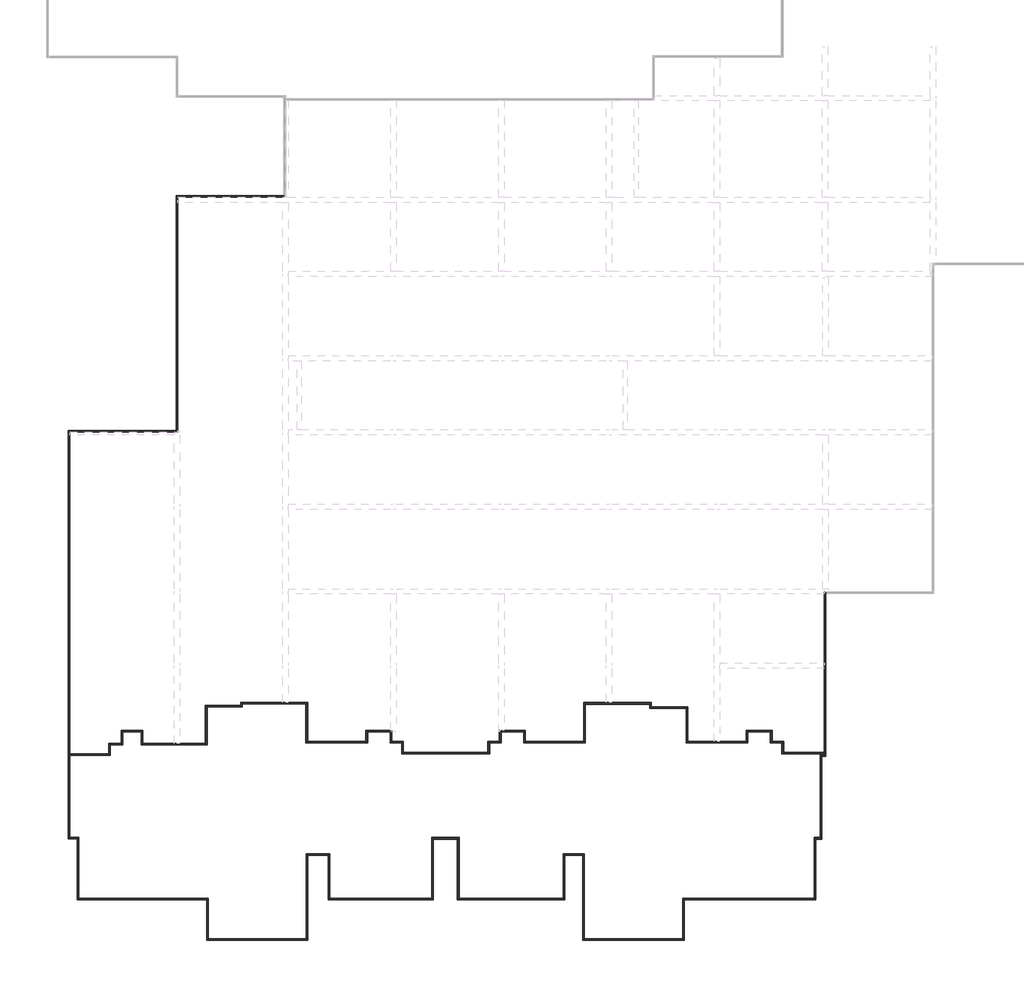
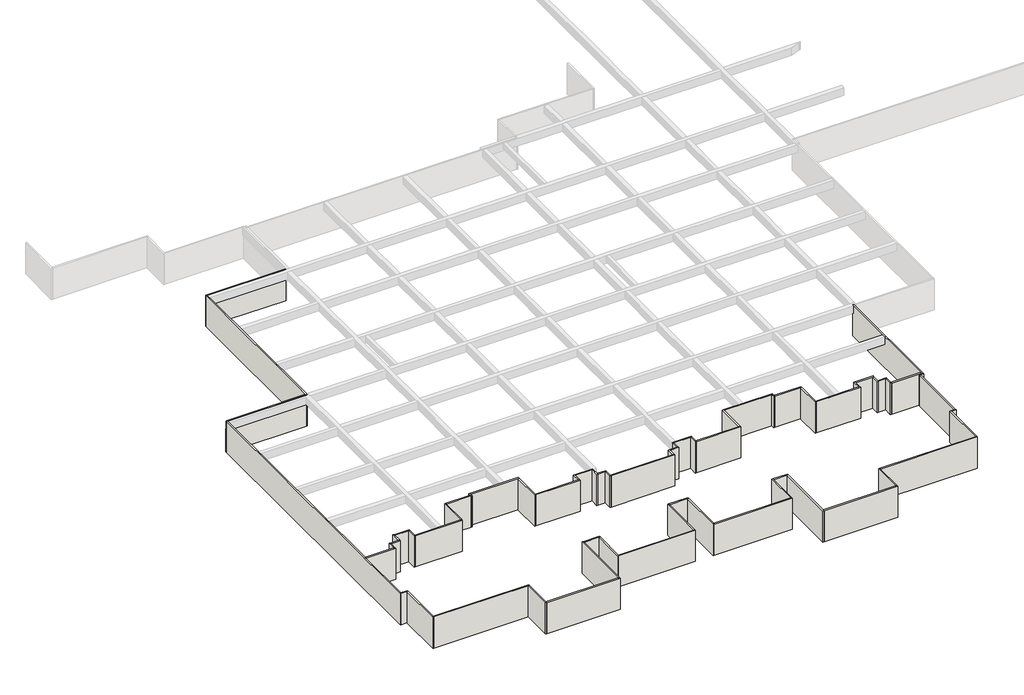
# One storey, part 1 of 14: 65 walls.
"""IFC4 building model written with IfcOpenShell, lengths in millimetres."""

from ifc_helpers import new_model, si_unit, origin, origin_with_axes, place, context, project, spatial, polyline, outline, extrude, faceted_brep, element, save

model = new_model("IFC4")

# Units and contexts
model_context = context("Model", 3, world=origin())
ifc_project = project(units=[si_unit("LENGTHUNIT", "METRE", prefix="MILLI")], contexts=[model_context])

# Site, building, storey
site = spatial("IfcSite", under=ifc_project)
building = spatial("IfcBuilding", under=site)
storey = spatial("IfcBuildingStorey", under=building, Name="户型图", Elevation=0.0)

# Walls
placement = place(None, origin())
element("IfcWall", 1, ObjectType="所有墙体", at=placement, inside=storey, context=model_context, shape_type="Brep", body=[
    faceted_brep([(-578191.2602569, -192711.2417661, 0.0), (-586191.2602569, -192711.2417661, 0.0), (-586191.2602569, -192711.2417661, 3300.0), (-578267.6529954, -192711.2417661, 3300.0), (-578191.2602569, -192711.2417661, 3300.0), (-578191.2602569, -192711.2417661, 2500.0), (-578191.2602569, -192831.2417661, 0.0), (-578191.2602569, -192831.2417661, 3300.0), (-578267.6529954, -192831.2417661, 3300.0), (-586071.2602569, -192831.2417661, 3300.0), (-586191.2602569, -192831.2417661, 3300.0), (-586191.2602569, -192831.2417661, 0.0), (-586071.2602569, -192831.2417661, 0.0)], [[[0, 1, 2, 3, 4, 5]], [[6, 7, 8, 9, 10, 11, 12]], [[1, 0, 6, 12, 11]], [[4, 3, 2, 10, 9, 8, 7]], [[0, 5, 4, 7, 6]], [[2, 1, 11, 10]]]),
])
element("IfcWall", 2, ObjectType="所有墙体", at=placement, inside=storey, context=model_context, shape_type="Brep", body=[
    faceted_brep([(-586191.2602569, -192831.2417661, 0.0), (-586191.2602569, -210132.8565135, 0.0), (-586191.2602569, -210252.8565135, 0.0), (-586191.2602569, -210252.8565135, 3300.0), (-586191.2602569, -210132.8565135, 3300.0), (-586191.2602569, -210092.8565135, 3300.0), (-586191.2602569, -192831.2417661, 3300.0), (-586071.2602569, -192831.2417661, 0.0), (-586071.2602569, -192831.2417661, 3300.0), (-586071.2602569, -210092.8565135, 3300.0), (-586071.2602569, -210132.8565135, 3300.0), (-586071.2602569, -210252.8565135, 3300.0), (-586071.2602569, -210252.8565135, 2500.0), (-586071.2602569, -210252.8565135, 0.0)], [[[0, 1, 2, 3, 4, 5, 6]], [[7, 8, 9, 10, 11, 12, 13]], [[2, 1, 0, 7, 13]], [[6, 5, 4, 3, 11, 10, 9, 8]], [[0, 6, 8, 7]], [[3, 2, 13, 12, 11]]]),
])
element("IfcWall", 3, ObjectType="所有墙体", at=placement, inside=storey, context=model_context, shape_type="Brep", body=[
    faceted_brep([(-586191.2602569, -210132.8565135, 0.0), (-594191.2602569, -210132.8565135, 0.0), (-594191.2602569, -210132.8565135, 3300.0), (-586191.2602569, -210132.8565135, 3300.0), (-586191.2602569, -210252.8565135, 0.0), (-586191.2602569, -210252.8565135, 3300.0), (-594071.2602569, -210252.8565135, 3300.0), (-594191.2602569, -210252.8565135, 3300.0), (-594191.2602569, -210252.8565135, 0.0), (-594071.2602569, -210252.8565135, 0.0)], [[[0, 1, 2, 3]], [[4, 5, 6, 7, 8, 9]], [[1, 0, 4, 9, 8]], [[3, 2, 7, 6, 5]], [[0, 3, 5, 4]], [[2, 1, 8, 7]]]),
])
element("IfcWall", 4, ObjectType="所有墙体", at=placement, inside=storey, context=model_context, shape_type="Brep", body=[
    faceted_brep([(-594191.2602569, -210252.8565135, 0.0), (-594191.2602569, -240452.8565135, 0.0), (-594191.2602569, -240452.8565135, 3300.0), (-594191.2602569, -210252.8565135, 3300.0), (-594071.2602569, -210252.8565135, 0.0), (-594071.2602569, -210252.8565135, 3300.0), (-594071.2602569, -234140.252781, 3300.0), (-594071.2602569, -234260.252781, 3300.0), (-594071.2602569, -240332.8565135, 3300.0), (-594071.2602569, -240452.8565135, 3300.0), (-594071.2602569, -240452.8565135, 0.0), (-594071.2602569, -240332.8565135, 0.0), (-594071.2602569, -234260.252781, 0.0), (-594071.2602569, -234140.252781, 0.0)], [[[0, 1, 2, 3]], [[4, 5, 6, 7, 8, 9, 10, 11, 12, 13]], [[1, 0, 4, 13, 12, 11, 10]], [[3, 2, 9, 8, 7, 6, 5]], [[0, 3, 5, 4]], [[2, 1, 10, 9]]]),
])
element("IfcWall", 5, ObjectType="所有墙体", at=placement, inside=storey, context=model_context, shape_type="Brep", body=[
    faceted_brep([(-594071.2602569, -240452.8565135, 0.0), (-593517.7604721, -240452.8565135, 0.0), (-593397.7604721, -240452.8565135, 0.0), (-593397.7604721, -240452.8565135, 3300.0), (-593517.7604721, -240452.8565135, 3300.0), (-594071.2602569, -240452.8565135, 3300.0), (-594071.2602569, -240332.8565135, 0.0), (-594071.2602569, -240332.8565135, 3300.0), (-593397.7604721, -240332.8565135, 3300.0), (-593397.7604721, -240332.8565135, 0.0)], [[[0, 1, 2, 3, 4, 5]], [[6, 7, 8, 9]], [[2, 1, 0, 6, 9]], [[5, 4, 3, 8, 7]], [[0, 5, 7, 6]], [[3, 2, 9, 8]]]),
])
element("IfcWall", 6, ObjectType="所有墙体", at=placement, inside=storey, context=model_context, shape_type="Brep", body=[
    faceted_brep([(-593517.7604721, -240452.8565135, 0.0), (-593517.7604721, -244961.010998, 0.0), (-593517.7604721, -244961.010998, 3300.0), (-593517.7604721, -240452.8565135, 3300.0), (-593397.7604721, -240452.8565135, 0.0), (-593397.7604721, -240452.8565135, 3300.0), (-593397.7604721, -244841.010998, 3300.0), (-593397.7604721, -244961.010998, 3300.0), (-593397.7604721, -244961.010998, 0.0), (-593397.7604721, -244841.010998, 0.0)], [[[0, 1, 2, 3]], [[4, 5, 6, 7, 8, 9]], [[1, 0, 4, 9, 8]], [[3, 2, 7, 6, 5]], [[0, 3, 5, 4]], [[2, 1, 8, 7]]]),
])
element("IfcWall", 7, ObjectType="所有墙体", at=placement, inside=storey, context=model_context, shape_type="Brep", body=[
    faceted_brep([(-593397.7604721, -244961.010998, 0.0), (-583922.7851213, -244961.010998, 0.0), (-583802.7851213, -244961.010998, 0.0), (-583802.7851213, -244961.010998, 3300.0), (-583922.7851213, -244961.010998, 3300.0), (-593397.7604721, -244961.010998, 3300.0), (-593397.7604721, -244841.010998, 0.0), (-593397.7604721, -244841.010998, 3300.0), (-583802.7851213, -244841.010998, 3300.0), (-583802.7851213, -244841.010998, 0.0)], [[[0, 1, 2, 3, 4, 5]], [[6, 7, 8, 9]], [[2, 1, 0, 6, 9]], [[5, 4, 3, 8, 7]], [[0, 5, 7, 6]], [[3, 2, 9, 8]]]),
])
element("IfcWall", 8, ObjectType="所有墙体", at=placement, inside=storey, context=model_context, shape_type="Brep", body=[
    faceted_brep([(-583922.7851213, -244961.010998, 0.0), (-583922.7851213, -247971.7198422, 0.0), (-583922.7851213, -247971.7198422, 3300.0), (-583922.7851213, -244961.010998, 3300.0), (-583802.7851213, -244961.010998, 0.0), (-583802.7851213, -244961.010998, 3300.0), (-583802.7851213, -247851.7198422, 3300.0), (-583802.7851213, -247971.7198422, 3300.0), (-583802.7851213, -247971.7198422, 0.0), (-583802.7851213, -247851.7198422, 0.0)], [[[0, 1, 2, 3]], [[4, 5, 6, 7, 8, 9]], [[1, 0, 4, 9, 8]], [[3, 2, 7, 6, 5]], [[0, 3, 5, 4]], [[2, 1, 8, 7]]]),
])
element("IfcWall", 9, ObjectType="所有墙体", at=placement, inside=storey, context=model_context, shape_type="Brep", body=[
    faceted_brep([(-583802.7851213, -247971.7198422, 0.0), (-576406.141893, -247971.7198422, 0.0), (-576406.141893, -247971.7198422, 3300.0), (-583802.7851213, -247971.7198422, 3300.0), (-583802.7851213, -247851.7198422, 0.0), (-583802.7851213, -247851.7198422, 3300.0), (-576526.141893, -247851.7198422, 3300.0), (-576406.141893, -247851.7198422, 3300.0), (-576406.141893, -247851.7198422, 0.0), (-576526.141893, -247851.7198422, 0.0)], [[[0, 1, 2, 3]], [[4, 5, 6, 7, 8, 9]], [[1, 0, 4, 9, 8]], [[3, 2, 7, 6, 5]], [[0, 3, 5, 4]], [[2, 1, 8, 7]]]),
])
element("IfcWall", 10, ObjectType="所有墙体", at=placement, inside=storey, context=model_context, shape_type="Brep", body=[
    faceted_brep([(-576406.141893, -247851.7198422, 0.0), (-576406.141893, -241679.9697972, 0.0), (-576406.141893, -241559.9697972, 0.0), (-576406.141893, -241559.9697972, 3300.0), (-576406.141893, -241679.9697972, 3300.0), (-576406.141893, -247851.7198422, 3300.0), (-576526.141893, -247851.7198422, 0.0), (-576526.141893, -247851.7198422, 3300.0), (-576526.141893, -241559.9697972, 3300.0), (-576526.141893, -241559.9697972, 0.0)], [[[0, 1, 2, 3, 4, 5]], [[6, 7, 8, 9]], [[2, 1, 0, 6, 9]], [[5, 4, 3, 8, 7]], [[0, 5, 7, 6]], [[3, 2, 9, 8]]]),
])
element("IfcWall", 11, ObjectType="所有墙体", at=placement, inside=storey, context=model_context, shape_type="Brep", body=[
    faceted_brep([(-576406.141893, -241679.9697972, 0.0), (-574919.1182202, -241679.9697972, 0.0), (-574799.1182202, -241679.9697972, 0.0), (-574799.1182202, -241679.9697972, 3300.0), (-574919.1182202, -241679.9697972, 3300.0), (-576406.141893, -241679.9697972, 3300.0), (-576406.141893, -241559.9697972, 0.0), (-576406.141893, -241559.9697972, 3300.0), (-574799.1182202, -241559.9697972, 3300.0), (-574799.1182202, -241559.9697972, 0.0)], [[[0, 1, 2, 3, 4, 5]], [[6, 7, 8, 9]], [[2, 1, 0, 6, 9]], [[5, 4, 3, 8, 7]], [[0, 5, 7, 6]], [[3, 2, 9, 8]]]),
])
element("IfcWall", 12, ObjectType="所有墙体", at=placement, inside=storey, context=model_context, shape_type="Brep", body=[
    faceted_brep([(-574919.1182202, -241679.9697972, 0.0), (-574919.1182202, -244961.010998, 0.0), (-574919.1182202, -244961.010998, 3300.0), (-574919.1182202, -241679.9697972, 3300.0), (-574799.1182202, -241679.9697972, 0.0), (-574799.1182202, -241679.9697972, 3300.0), (-574799.1182202, -244841.010998, 3300.0), (-574799.1182202, -244961.010998, 3300.0), (-574799.1182202, -244961.010998, 0.0), (-574799.1182202, -244841.010998, 0.0)], [[[0, 1, 2, 3]], [[4, 5, 6, 7, 8, 9]], [[1, 0, 4, 9, 8]], [[3, 2, 7, 6, 5]], [[0, 3, 5, 4]], [[2, 1, 8, 7]]]),
])
element("IfcWall", 13, ObjectType="所有墙体", at=placement, inside=storey, context=model_context, shape_type="Brep", body=[
    faceted_brep([(-574799.1182202, -244961.010998, 0.0), (-567099.1182202, -244961.010998, 0.0), (-567099.1182202, -244961.010998, 3300.0), (-574799.1182202, -244961.010998, 3300.0), (-574799.1182202, -244841.010998, 0.0), (-574799.1182202, -244841.010998, 3300.0), (-567219.1182202, -244841.010998, 3300.0), (-567099.1182202, -244841.010998, 3300.0), (-567099.1182202, -244841.010998, 0.0), (-567219.1182202, -244841.010998, 0.0)], [[[0, 1, 2, 3]], [[4, 5, 6, 7, 8, 9]], [[1, 0, 4, 9, 8]], [[3, 2, 7, 6, 5]], [[0, 3, 5, 4]], [[2, 1, 8, 7]]]),
])
element("IfcWall", 14, ObjectType="所有墙体", at=placement, inside=storey, context=model_context, shape_type="Brep", body=[
    faceted_brep([(-567099.1182202, -244841.010998, 0.0), (-567099.1182202, -240461.010998, 0.0), (-567099.1182202, -240341.010998, 0.0), (-567099.1182202, -240341.010998, 3300.0), (-567099.1182202, -240461.010998, 3300.0), (-567099.1182202, -244841.010998, 3300.0), (-567219.1182202, -244841.010998, 0.0), (-567219.1182202, -244841.010998, 3300.0), (-567219.1182202, -240341.010998, 3300.0), (-567219.1182202, -240341.010998, 0.0)], [[[0, 1, 2, 3, 4, 5]], [[6, 7, 8, 9]], [[2, 1, 0, 6, 9]], [[5, 4, 3, 8, 7]], [[0, 5, 7, 6]], [[3, 2, 9, 8]]]),
])
element("IfcWall", 15, ObjectType="所有墙体", at=placement, inside=storey, context=model_context, shape_type="Brep", body=[
    faceted_brep([(-567099.1182202, -240461.010998, 0.0), (-565319.1182202, -240461.010998, 0.0), (-565199.1182202, -240461.010998, 0.0), (-565199.1182202, -240461.010998, 3300.0), (-565319.1182202, -240461.010998, 3300.0), (-567099.1182202, -240461.010998, 3300.0), (-567099.1182202, -240341.010998, 0.0), (-567099.1182202, -240341.010998, 3300.0), (-565199.1182202, -240341.010998, 3300.0), (-565199.1182202, -240341.010998, 0.0)], [[[0, 1, 2, 3, 4, 5]], [[6, 7, 8, 9]], [[2, 1, 0, 6, 9]], [[5, 4, 3, 8, 7]], [[0, 5, 7, 6]], [[3, 2, 9, 8]]]),
])
element("IfcWall", 16, ObjectType="所有墙体", at=placement, inside=storey, context=model_context, shape_type="Brep", body=[
    faceted_brep([(-565319.1182202, -240461.010998, 0.0), (-565319.1182202, -244961.010998, 0.0), (-565319.1182202, -244961.010998, 3300.0), (-565319.1182202, -240461.010998, 3300.0), (-565199.1182202, -240461.010998, 0.0), (-565199.1182202, -240461.010998, 3300.0), (-565199.1182202, -244841.010998, 3300.0), (-565199.1182202, -244961.010998, 3300.0), (-565199.1182202, -244961.010998, 0.0), (-565199.1182202, -244841.010998, 0.0)], [[[0, 1, 2, 3]], [[4, 5, 6, 7, 8, 9]], [[1, 0, 4, 9, 8]], [[3, 2, 7, 6, 5]], [[0, 3, 5, 4]], [[2, 1, 8, 7]]]),
])
element("IfcWall", 17, ObjectType="所有墙体", at=placement, inside=storey, context=model_context, shape_type="Brep", body=[
    faceted_brep([(-565199.1182202, -244961.010998, 0.0), (-557352.768648, -244961.010998, 0.0), (-557352.768648, -244961.010998, 3300.0), (-565199.1182202, -244961.010998, 3300.0), (-565199.1182202, -244841.010998, 0.0), (-565199.1182202, -244841.010998, 3300.0), (-557472.768648, -244841.010998, 3300.0), (-557352.768648, -244841.010998, 3300.0), (-557352.768648, -244841.010998, 0.0), (-557472.768648, -244841.010998, 0.0)], [[[0, 1, 2, 3]], [[4, 5, 6, 7, 8, 9]], [[1, 0, 4, 9, 8]], [[3, 2, 7, 6, 5]], [[0, 3, 5, 4]], [[2, 1, 8, 7]]]),
])
element("IfcWall", 18, ObjectType="所有墙体", at=placement, inside=storey, context=model_context, shape_type="Brep", body=[
    faceted_brep([(-557352.768648, -244841.010998, 0.0), (-557352.768648, -241679.9697972, 0.0), (-557352.768648, -241559.9697972, 0.0), (-557352.768648, -241559.9697972, 3300.0), (-557352.768648, -241679.9697972, 3300.0), (-557352.768648, -244841.010998, 3300.0), (-557472.768648, -244841.010998, 0.0), (-557472.768648, -244841.010998, 3300.0), (-557472.768648, -241559.9697972, 3300.0), (-557472.768648, -241559.9697972, 0.0)], [[[0, 1, 2, 3, 4, 5]], [[6, 7, 8, 9]], [[2, 1, 0, 6, 9]], [[5, 4, 3, 8, 7]], [[0, 5, 7, 6]], [[3, 2, 9, 8]]]),
])
element("IfcWall", 19, ObjectType="所有墙体", at=placement, inside=storey, context=model_context, shape_type="Brep", body=[
    faceted_brep([(-557352.768648, -241679.9697972, 0.0), (-556019.1064476, -241679.9697972, 0.0), (-555899.1064476, -241679.9697972, 0.0), (-555899.1064476, -241679.9697972, 3300.0), (-556019.1064476, -241679.9697972, 3300.0), (-557352.768648, -241679.9697972, 3300.0), (-557352.768648, -241559.9697972, 0.0), (-557352.768648, -241559.9697972, 3300.0), (-555899.1064476, -241559.9697972, 3300.0), (-555899.1064476, -241559.9697972, 0.0)], [[[0, 1, 2, 3, 4, 5]], [[6, 7, 8, 9]], [[2, 1, 0, 6, 9]], [[5, 4, 3, 8, 7]], [[0, 5, 7, 6]], [[3, 2, 9, 8]]]),
])
element("IfcWall", 20, ObjectType="所有墙体", at=placement, inside=storey, context=model_context, shape_type="Brep", body=[
    faceted_brep([(-556019.1064476, -241679.9697972, 0.0), (-556019.1064476, -247971.7198422, 0.0), (-556019.1064476, -247971.7198422, 3300.0), (-556019.1064476, -241679.9697972, 3300.0), (-555899.1064476, -241679.9697972, 0.0), (-555899.1064476, -241679.9697972, 3300.0), (-555899.1064476, -247851.7198422, 3300.0), (-555899.1064476, -247971.7198422, 3300.0), (-555899.1064476, -247971.7198422, 0.0), (-555899.1064476, -247851.7198422, 0.0)], [[[0, 1, 2, 3]], [[4, 5, 6, 7, 8, 9]], [[1, 0, 4, 9, 8]], [[3, 2, 7, 6, 5]], [[0, 3, 5, 4]], [[2, 1, 8, 7]]]),
])
element("IfcWall", 21, ObjectType="所有墙体", at=placement, inside=storey, context=model_context, shape_type="Brep", body=[
    faceted_brep([(-555899.1064476, -247971.7198422, 0.0), (-548506.1227729, -247971.7198422, 0.0), (-548506.1227729, -247971.7198422, 3300.0), (-555899.1064476, -247971.7198422, 3300.0), (-555899.1064476, -247851.7198422, 0.0), (-555899.1064476, -247851.7198422, 3300.0), (-548626.1227729, -247851.7198422, 3300.0), (-548506.1227729, -247851.7198422, 3300.0), (-548506.1227729, -247851.7198422, 0.0), (-548626.1227729, -247851.7198422, 0.0)], [[[0, 1, 2, 3]], [[4, 5, 6, 7, 8, 9]], [[1, 0, 4, 9, 8]], [[3, 2, 7, 6, 5]], [[0, 3, 5, 4]], [[2, 1, 8, 7]]]),
])
element("IfcWall", 22, ObjectType="所有墙体", at=placement, inside=storey, context=model_context, shape_type="Brep", body=[
    faceted_brep([(-548506.1227729, -247851.7198422, 0.0), (-548506.1227729, -244961.010998, 0.0), (-548506.1227729, -244841.010998, 0.0), (-548506.1227729, -244841.010998, 3300.0), (-548506.1227729, -244961.010998, 3300.0), (-548506.1227729, -247851.7198422, 3300.0), (-548626.1227729, -247851.7198422, 0.0), (-548626.1227729, -247851.7198422, 3300.0), (-548626.1227729, -244841.010998, 3300.0), (-548626.1227729, -244841.010998, 0.0)], [[[0, 1, 2, 3, 4, 5]], [[6, 7, 8, 9]], [[2, 1, 0, 6, 9]], [[5, 4, 3, 8, 7]], [[0, 5, 7, 6]], [[3, 2, 9, 8]]]),
])
element("IfcWall", 23, ObjectType="所有墙体", at=placement, inside=storey, context=model_context, shape_type="Brep", body=[
    faceted_brep([(-548506.1227729, -244961.010998, 0.0), (-538752.7570659, -244961.010998, 0.0), (-538752.7570659, -244961.010998, 3300.0), (-548506.1227729, -244961.010998, 3300.0), (-548506.1227729, -244841.010998, 0.0), (-548506.1227729, -244841.010998, 3300.0), (-538872.7570659, -244841.010998, 3300.0), (-538752.7570659, -244841.010998, 3300.0), (-538752.7570659, -244841.010998, 0.0), (-538872.7570659, -244841.010998, 0.0)], [[[0, 1, 2, 3]], [[4, 5, 6, 7, 8, 9]], [[1, 0, 4, 9, 8]], [[3, 2, 7, 6, 5]], [[0, 3, 5, 4]], [[2, 1, 8, 7]]]),
])
element("IfcWall", 24, ObjectType="所有墙体", at=placement, inside=storey, context=model_context, shape_type="Brep", body=[
    faceted_brep([(-538752.7570659, -244841.010998, 0.0), (-538752.7570659, -240461.010998, 0.0), (-538752.7570659, -240341.010998, 0.0), (-538752.7570659, -240341.010998, 3300.0), (-538752.7570659, -240461.010998, 3300.0), (-538752.7570659, -244841.010998, 3300.0), (-538872.7570659, -244841.010998, 0.0), (-538872.7570659, -244841.010998, 3300.0), (-538872.7570659, -240341.010998, 3300.0), (-538872.7570659, -240341.010998, 0.0)], [[[0, 1, 2, 3, 4, 5]], [[6, 7, 8, 9]], [[2, 1, 0, 6, 9]], [[5, 4, 3, 8, 7]], [[0, 5, 7, 6]], [[3, 2, 9, 8]]]),
])
element("IfcWall", 25, ObjectType="所有墙体", at=placement, inside=storey, context=model_context, shape_type="Brep", body=[
    faceted_brep([(-538752.7570659, -240461.010998, 0.0), (-538297.7352575, -240461.010998, 0.0), (-538297.7352575, -240461.010998, 3300.0), (-538752.7570659, -240461.010998, 3300.0), (-538752.7570659, -240341.010998, 0.0), (-538752.7570659, -240341.010998, 3300.0), (-538417.7352575, -240341.010998, 3300.0), (-538297.7352575, -240341.010998, 3300.0), (-538297.7352575, -240341.010998, 0.0), (-538417.7352575, -240341.010998, 0.0)], [[[0, 1, 2, 3]], [[4, 5, 6, 7, 8, 9]], [[1, 0, 4, 9, 8]], [[3, 2, 7, 6, 5]], [[0, 3, 5, 4]], [[2, 1, 8, 7]]]),
])
element("IfcWall", 26, ObjectType="所有墙体", at=placement, inside=storey, context=model_context, shape_type="SweptSolid", body=[
    extrude(outline(polyline([(-538297.7352575, -234322.4901809), (-538297.7352575, -240341.010998), (-538417.7352575, -240341.010998), (-538417.7352575, -234322.4901809), (-538297.7352575, -234322.4901809)])), origin_with_axes(), (0.0, 0.0, 1.0), 3300.0),
])
element("IfcWall", 27, ObjectType="所有墙体", at=placement, inside=storey, context=model_context, shape_type="Brep", body=[
    faceted_brep([(-538417.7352575, -234322.4901809, 0.0), (-538297.7352575, -234322.4901809, 0.0), (-537997.7352575, -234322.4901809, 0.0), (-537997.7352575, -234322.4901809, 3300.0), (-538297.7352575, -234322.4901809, 3300.0), (-538417.7352575, -234322.4901809, 3300.0), (-538417.7352575, -234202.4901809, 0.0), (-538417.7352575, -234202.4901809, 3300.0), (-538117.7352575, -234202.4901809, 3300.0), (-537997.7352575, -234202.4901809, 3300.0), (-537997.7352575, -234202.4901809, 0.0), (-538117.7352575, -234202.4901809, 0.0)], [[[0, 1, 2, 3, 4, 5]], [[6, 7, 8, 9, 10, 11]], [[2, 1, 0, 6, 11, 10]], [[5, 4, 3, 9, 8, 7]], [[0, 5, 7, 6]], [[3, 2, 10, 9]]]),
])
element("IfcWall", 28, ObjectType="所有墙体", at=placement, inside=storey, context=model_context, shape_type="Brep", body=[
    faceted_brep([(-537997.7352575, -234202.4901809, 0.0), (-537997.7352575, -222250.9174567, 0.0), (-537997.7352575, -222130.9174567, 0.0), (-537997.7352575, -222130.9174567, 3300.0), (-537997.7352575, -222250.9174567, 3300.0), (-537997.7352575, -222292.8565135, 3300.0), (-537997.7352575, -234202.4901809, 3300.0), (-538117.7352575, -234202.4901809, 0.0), (-538117.7352575, -234202.4901809, 3300.0), (-538117.7352575, -234137.8504047, 3300.0), (-538117.7352575, -234017.8504047, 3300.0), (-538117.7352575, -222292.8565135, 3300.0), (-538117.7352575, -222130.9174567, 3300.0), (-538117.7352575, -222130.9174567, 2500.0), (-538117.7352575, -222130.9174567, 0.0), (-538117.7352575, -234017.8504047, 0.0), (-538117.7352575, -234137.8504047, 0.0)], [[[0, 1, 2, 3, 4, 5, 6]], [[7, 8, 9, 10, 11, 12, 13, 14, 15, 16]], [[2, 1, 0, 7, 16, 15, 14]], [[6, 5, 4, 3, 12, 11, 10, 9, 8]], [[0, 6, 8, 7]], [[3, 2, 14, 13, 12]]]),
])
element("IfcWall", 29, ObjectType="所有墙体", at=placement, inside=storey, context=model_context, shape_type="Brep", body=[
    faceted_brep([(-594071.2602569, -234260.252781, 0.0), (-591071.2602569, -234260.252781, 0.0), (-591071.2602569, -234260.252781, 3300.0), (-594071.2602569, -234260.252781, 3300.0), (-594071.2602569, -234140.252781, 0.0), (-594071.2602569, -234140.252781, 3300.0), (-591191.2602569, -234140.252781, 3300.0), (-591071.2602569, -234140.252781, 3300.0), (-591071.2602569, -234140.252781, 0.0), (-591191.2602569, -234140.252781, 0.0)], [[[0, 1, 2, 3]], [[4, 5, 6, 7, 8, 9]], [[1, 0, 4, 9, 8]], [[3, 2, 7, 6, 5]], [[0, 3, 5, 4]], [[2, 1, 8, 7]]]),
])
element("IfcWall", 30, ObjectType="所有墙体", at=placement, inside=storey, context=model_context, shape_type="Brep", body=[
    faceted_brep([(-591071.2602569, -234140.252781, 0.0), (-591071.2602569, -233463.599968, 0.0), (-591071.2602569, -233343.599968, 0.0), (-591071.2602569, -233343.599968, 3300.0), (-591071.2602569, -233463.599968, 3300.0), (-591071.2602569, -234140.252781, 3300.0), (-591191.2602569, -234140.252781, 0.0), (-591191.2602569, -234140.252781, 3300.0), (-591191.2602569, -233343.599968, 3300.0), (-591191.2602569, -233343.599968, 0.0)], [[[0, 1, 2, 3, 4, 5]], [[6, 7, 8, 9]], [[2, 1, 0, 6, 9]], [[5, 4, 3, 8, 7]], [[0, 5, 7, 6]], [[3, 2, 9, 8]]]),
])
element("IfcWall", 31, ObjectType="所有墙体", at=placement, inside=storey, context=model_context, shape_type="Brep", body=[
    faceted_brep([(-591071.2602569, -233463.599968, 0.0), (-590139.9591732, -233463.599968, 0.0), (-590139.9591732, -233463.599968, 3300.0), (-591071.2602569, -233463.599968, 3300.0), (-591071.2602569, -233343.599968, 0.0), (-591071.2602569, -233343.599968, 3300.0), (-590259.9591732, -233343.599968, 3300.0), (-590139.9591732, -233343.599968, 3300.0), (-590139.9591732, -233343.599968, 0.0), (-590259.9591732, -233343.599968, 0.0)], [[[0, 1, 2, 3]], [[4, 5, 6, 7, 8, 9]], [[1, 0, 4, 9, 8]], [[3, 2, 7, 6, 5]], [[0, 3, 5, 4]], [[2, 1, 8, 7]]]),
])
element("IfcWall", 32, ObjectType="所有墙体", at=placement, inside=storey, context=model_context, shape_type="Brep", body=[
    faceted_brep([(-590139.9591732, -233343.599968, 0.0), (-590139.9591732, -232514.6386108, 0.0), (-590139.9591732, -232394.6386108, 0.0), (-590139.9591732, -232394.6386108, 3300.0), (-590139.9591732, -232514.6386108, 3300.0), (-590139.9591732, -233343.599968, 3300.0), (-590259.9591732, -233343.599968, 0.0), (-590259.9591732, -233343.599968, 3300.0), (-590259.9591732, -232394.6386108, 3300.0), (-590259.9591732, -232394.6386108, 0.0)], [[[0, 1, 2, 3, 4, 5]], [[6, 7, 8, 9]], [[2, 1, 0, 6, 9]], [[5, 4, 3, 8, 7]], [[0, 5, 7, 6]], [[3, 2, 9, 8]]]),
])
element("IfcWall", 33, ObjectType="所有墙体", at=placement, inside=storey, context=model_context, shape_type="Brep", body=[
    faceted_brep([(-590139.9591732, -232514.6386108, 0.0), (-588758.8992985, -232514.6386108, 0.0), (-588638.8992985, -232514.6386108, 0.0), (-588638.8992985, -232514.6386108, 3300.0), (-588758.8992985, -232514.6386108, 3300.0), (-590139.9591732, -232514.6386108, 3300.0), (-590139.9591732, -232394.6386108, 0.0), (-590139.9591732, -232394.6386108, 3300.0), (-588638.8992985, -232394.6386108, 3300.0), (-588638.8992985, -232394.6386108, 0.0)], [[[0, 1, 2, 3, 4, 5]], [[6, 7, 8, 9]], [[2, 1, 0, 6, 9]], [[5, 4, 3, 8, 7]], [[0, 5, 7, 6]], [[3, 2, 9, 8]]]),
])
element("IfcWall", 34, ObjectType="所有墙体", at=placement, inside=storey, context=model_context, shape_type="Brep", body=[
    faceted_brep([(-588758.8992985, -232514.6386108, 0.0), (-588758.8992985, -233463.599968, 0.0), (-588758.8992985, -233463.599968, 3300.0), (-588758.8992985, -232514.6386108, 3300.0), (-588638.8992985, -232514.6386108, 0.0), (-588638.8992985, -232514.6386108, 3300.0), (-588638.8992985, -233343.599968, 3300.0), (-588638.8992985, -233463.599968, 3300.0), (-588638.8992985, -233463.599968, 0.0), (-588638.8992985, -233343.599968, 0.0)], [[[0, 1, 2, 3]], [[4, 5, 6, 7, 8, 9]], [[1, 0, 4, 9, 8]], [[3, 2, 7, 6, 5]], [[0, 3, 5, 4]], [[2, 1, 8, 7]]]),
])
element("IfcWall", 35, ObjectType="所有墙体", at=placement, inside=storey, context=model_context, shape_type="Brep", body=[
    faceted_brep([(-588638.8992985, -233463.599968, 0.0), (-583889.9552825, -233463.599968, 0.0), (-583889.9552825, -233463.599968, 3300.0), (-588638.8992985, -233463.599968, 3300.0), (-588638.8992985, -233343.599968, 0.0), (-588638.8992985, -233343.599968, 3300.0), (-584009.9552825, -233343.599968, 3300.0), (-583889.9552825, -233343.599968, 3300.0), (-583889.9552825, -233343.599968, 0.0), (-584009.9552825, -233343.599968, 0.0)], [[[0, 1, 2, 3]], [[4, 5, 6, 7, 8, 9]], [[1, 0, 4, 9, 8]], [[3, 2, 7, 6, 5]], [[0, 3, 5, 4]], [[2, 1, 8, 7]]]),
])
element("IfcWall", 36, ObjectType="所有墙体", at=placement, inside=storey, context=model_context, shape_type="Brep", body=[
    faceted_brep([(-583889.9552825, -233343.599968, 0.0), (-583889.9552825, -230671.6117982, 0.0), (-583889.9552825, -230551.6117982, 0.0), (-583889.9552825, -230551.6117982, 3300.0), (-583889.9552825, -230671.6117982, 3300.0), (-583889.9552825, -233343.599968, 3300.0), (-584009.9552825, -233343.599968, 0.0), (-584009.9552825, -233343.599968, 3300.0), (-584009.9552825, -230551.6117982, 3300.0), (-584009.9552825, -230551.6117982, 0.0)], [[[0, 1, 2, 3, 4, 5]], [[6, 7, 8, 9]], [[2, 1, 0, 6, 9]], [[5, 4, 3, 8, 7]], [[0, 5, 7, 6]], [[3, 2, 9, 8]]]),
])
element("IfcWall", 37, ObjectType="所有墙体", at=placement, inside=storey, context=model_context, shape_type="SweptSolid", body=[
    extrude(outline(polyline([(-581406.838098, -230671.6117982), (-583889.9552825, -230671.6117982), (-583889.9552825, -230551.6117982), (-581406.838098, -230551.6117982), (-581406.838098, -230671.6117982)])), origin_with_axes(), (0.0, 0.0, 1.0), 3300.0),
])
element("IfcWall", 38, ObjectType="所有墙体", at=placement, inside=storey, context=model_context, shape_type="Brep", body=[
    faceted_brep([(-581286.838098, -230671.6117982, 0.0), (-581286.838098, -230424.5164481, 0.0), (-581286.838098, -230304.5164481, 0.0), (-581286.838098, -230304.5164481, 3300.0), (-581286.838098, -230424.5164481, 3300.0), (-581286.838098, -230671.6117982, 3300.0), (-581406.838098, -230671.6117982, 0.0), (-581406.838098, -230671.6117982, 3300.0), (-581406.838098, -230551.6117982, 3300.0), (-581406.838098, -230304.5164481, 3300.0), (-581406.838098, -230304.5164481, 0.0), (-581406.838098, -230551.6117982, 0.0)], [[[0, 1, 2, 3, 4, 5]], [[6, 7, 8, 9, 10, 11]], [[2, 1, 0, 6, 11, 10]], [[5, 4, 3, 9, 8, 7]], [[0, 5, 7, 6]], [[3, 2, 10, 9]]]),
])
element("IfcWall", 39, ObjectType="所有墙体", at=placement, inside=storey, context=model_context, shape_type="Brep", body=[
    faceted_brep([(-581286.838098, -230424.5164481, 0.0), (-576556.5593395, -230424.5164481, 0.0), (-576436.5593395, -230424.5164481, 0.0), (-576436.5593395, -230424.5164481, 3300.0), (-576556.5593395, -230424.5164481, 3300.0), (-581286.838098, -230424.5164481, 3300.0), (-581286.838098, -230304.5164481, 0.0), (-581286.838098, -230304.5164481, 3300.0), (-576436.5593395, -230304.5164481, 3300.0), (-576436.5593395, -230304.5164481, 0.0)], [[[0, 1, 2, 3, 4, 5]], [[6, 7, 8, 9]], [[2, 1, 0, 6, 9]], [[5, 4, 3, 8, 7]], [[0, 5, 7, 6]], [[3, 2, 9, 8]]]),
])
element("IfcWall", 40, ObjectType="所有墙体", at=placement, inside=storey, context=model_context, shape_type="Brep", body=[
    faceted_brep([(-576556.5593395, -230424.5164481, 0.0), (-576556.5593395, -233329.9306648, 0.0), (-576556.5593395, -233329.9306648, 3300.0), (-576556.5593395, -230424.5164481, 3300.0), (-576436.5593395, -230424.5164481, 0.0), (-576436.5593395, -230424.5164481, 3300.0), (-576436.5593395, -233209.9306648, 3300.0), (-576436.5593395, -233329.9306648, 3300.0), (-576436.5593395, -233329.9306648, 0.0), (-576436.5593395, -233209.9306648, 0.0)], [[[0, 1, 2, 3]], [[4, 5, 6, 7, 8, 9]], [[1, 0, 4, 9, 8]], [[3, 2, 7, 6, 5]], [[0, 3, 5, 4]], [[2, 1, 8, 7]]]),
])
element("IfcWall", 41, ObjectType="所有墙体", at=placement, inside=storey, context=model_context, shape_type="Brep", body=[
    faceted_brep([(-576436.5593395, -233329.9306648, 0.0), (-571989.7987118, -233329.9306648, 0.0), (-571989.7987118, -233329.9306648, 3300.0), (-576436.5593395, -233329.9306648, 3300.0), (-576436.5593395, -233209.9306648, 0.0), (-576436.5593395, -233209.9306648, 3300.0), (-572109.7987118, -233209.9306648, 3300.0), (-571989.7987118, -233209.9306648, 3300.0), (-571989.7987118, -233209.9306648, 0.0), (-572109.7987118, -233209.9306648, 0.0)], [[[0, 1, 2, 3]], [[4, 5, 6, 7, 8, 9]], [[1, 0, 4, 9, 8]], [[3, 2, 7, 6, 5]], [[0, 3, 5, 4]], [[2, 1, 8, 7]]]),
])
element("IfcWall", 42, ObjectType="所有墙体", at=placement, inside=storey, context=model_context, shape_type="Brep", body=[
    faceted_brep([(-571989.7987118, -233209.9306648, 0.0), (-571989.7987118, -232514.6386108, 0.0), (-571989.7987118, -232394.6386108, 0.0), (-571989.7987118, -232394.6386108, 3300.0), (-571989.7987118, -232514.6386108, 3300.0), (-571989.7987118, -233209.9306648, 3300.0), (-572109.7987118, -233209.9306648, 0.0), (-572109.7987118, -233209.9306648, 3300.0), (-572109.7987118, -232394.6386108, 3300.0), (-572109.7987118, -232394.6386108, 0.0)], [[[0, 1, 2, 3, 4, 5]], [[6, 7, 8, 9]], [[2, 1, 0, 6, 9]], [[5, 4, 3, 8, 7]], [[0, 5, 7, 6]], [[3, 2, 9, 8]]]),
])
element("IfcWall", 43, ObjectType="所有墙体", at=placement, inside=storey, context=model_context, shape_type="Brep", body=[
    faceted_brep([(-571989.7987118, -232514.6386108, 0.0), (-570308.8878112, -232514.6386108, 0.0), (-570188.8878112, -232514.6386108, 0.0), (-570188.8878112, -232514.6386108, 3300.0), (-570308.8878112, -232514.6386108, 3300.0), (-571989.7987118, -232514.6386108, 3300.0), (-571989.7987118, -232394.6386108, 0.0), (-571989.7987118, -232394.6386108, 3300.0), (-570267.6529954, -232394.6386108, 3300.0), (-570188.8878112, -232394.6386108, 3300.0), (-570188.8878112, -232394.6386108, 2500.0), (-570188.8878112, -232394.6386108, 0.0)], [[[0, 1, 2, 3, 4, 5]], [[6, 7, 8, 9, 10, 11]], [[2, 1, 0, 6, 11]], [[5, 4, 3, 9, 8, 7]], [[0, 5, 7, 6]], [[3, 2, 11, 10, 9]]]),
])
element("IfcWall", 44, ObjectType="所有墙体", at=placement, inside=storey, context=model_context, shape_type="Brep", body=[
    faceted_brep([(-570308.8878112, -232514.6386108, 0.0), (-570308.8878112, -233329.9306648, 0.0), (-570308.8878112, -233329.9306648, 3300.0), (-570308.8878112, -232514.6386108, 3300.0), (-570188.8878112, -232514.6386108, 0.0), (-570188.8878112, -232514.6386108, 3300.0), (-570188.8878112, -233209.9306648, 3300.0), (-570188.8878112, -233329.9306648, 3300.0), (-570188.8878112, -233329.9306648, 0.0), (-570188.8878112, -233209.9306648, 0.0)], [[[0, 1, 2, 3]], [[4, 5, 6, 7, 8, 9]], [[1, 0, 4, 9, 8]], [[3, 2, 7, 6, 5]], [[0, 3, 5, 4]], [[2, 1, 8, 7]]]),
])
element("IfcWall", 45, ObjectType="所有墙体", at=placement, inside=storey, context=model_context, shape_type="Brep", body=[
    faceted_brep([(-570188.8878112, -233329.9306648, 0.0), (-569459.7970552, -233329.9306648, 0.0), (-569339.7970552, -233329.9306648, 0.0), (-569339.7970552, -233329.9306648, 3300.0), (-569459.7970552, -233329.9306648, 3300.0), (-570188.8878112, -233329.9306648, 3300.0), (-570188.8878112, -233209.9306648, 0.0), (-570188.8878112, -233209.9306648, 3300.0), (-569339.7970552, -233209.9306648, 3300.0), (-569339.7970552, -233209.9306648, 0.0)], [[[0, 1, 2, 3, 4, 5]], [[6, 7, 8, 9]], [[2, 1, 0, 6, 9]], [[5, 4, 3, 8, 7]], [[0, 5, 7, 6]], [[3, 2, 9, 8]]]),
])
element("IfcWall", 46, ObjectType="所有墙体", at=placement, inside=storey, context=model_context, shape_type="Brep", body=[
    faceted_brep([(-569459.7970552, -233329.9306648, 0.0), (-569459.7970552, -234137.8504047, 0.0), (-569459.7970552, -234137.8504047, 3300.0), (-569459.7970552, -233329.9306648, 3300.0), (-569339.7970552, -233329.9306648, 0.0), (-569339.7970552, -233329.9306648, 3300.0), (-569339.7970552, -234017.8504047, 3300.0), (-569339.7970552, -234137.8504047, 3300.0), (-569339.7970552, -234137.8504047, 0.0), (-569339.7970552, -234017.8504047, 0.0)], [[[0, 1, 2, 3]], [[4, 5, 6, 7, 8, 9]], [[1, 0, 4, 9, 8]], [[3, 2, 7, 6, 5]], [[0, 3, 5, 4]], [[2, 1, 8, 7]]]),
])
element("IfcWall", 47, ObjectType="所有墙体", at=placement, inside=storey, context=model_context, shape_type="Brep", body=[
    faceted_brep([(-569339.7970552, -234137.8504047, 0.0), (-562940.6946279, -234137.8504047, 0.0), (-562940.6946279, -234137.8504047, 3300.0), (-569339.7970552, -234137.8504047, 3300.0), (-569339.7970552, -234017.8504047, 0.0), (-569339.7970552, -234017.8504047, 3300.0), (-563060.6946279, -234017.8504047, 3300.0), (-562940.6946279, -234017.8504047, 3300.0), (-562940.6946279, -234017.8504047, 0.0), (-563060.6946279, -234017.8504047, 0.0)], [[[0, 1, 2, 3]], [[4, 5, 6, 7, 8, 9]], [[1, 0, 4, 9, 8]], [[3, 2, 7, 6, 5]], [[0, 3, 5, 4]], [[2, 1, 8, 7]]]),
])
element("IfcWall", 48, ObjectType="所有墙体", at=placement, inside=storey, context=model_context, shape_type="Brep", body=[
    faceted_brep([(-562940.6946279, -234017.8504047, 0.0), (-562940.6946279, -233329.9306648, 0.0), (-562940.6946279, -233209.9306648, 0.0), (-562940.6946279, -233209.9306648, 3300.0), (-562940.6946279, -233329.9306648, 3300.0), (-562940.6946279, -234017.8504047, 3300.0), (-563060.6946279, -234017.8504047, 0.0), (-563060.6946279, -234017.8504047, 3300.0), (-563060.6946279, -233209.9306648, 3300.0), (-563060.6946279, -233209.9306648, 0.0)], [[[0, 1, 2, 3, 4, 5]], [[6, 7, 8, 9]], [[2, 1, 0, 6, 9]], [[5, 4, 3, 8, 7]], [[0, 5, 7, 6]], [[3, 2, 9, 8]]]),
])
element("IfcWall", 49, ObjectType="所有墙体", at=placement, inside=storey, context=model_context, shape_type="Brep", body=[
    faceted_brep([(-562940.6946279, -233329.9306648, 0.0), (-562089.7925406, -233329.9306648, 0.0), (-562089.7925406, -233329.9306648, 3300.0), (-562940.6946279, -233329.9306648, 3300.0), (-562940.6946279, -233209.9306648, 0.0), (-562940.6946279, -233209.9306648, 3300.0), (-562209.7925406, -233209.9306648, 3300.0), (-562089.7925406, -233209.9306648, 3300.0), (-562089.7925406, -233209.9306648, 0.0), (-562209.7925406, -233209.9306648, 0.0)], [[[0, 1, 2, 3]], [[4, 5, 6, 7, 8, 9]], [[1, 0, 4, 9, 8]], [[3, 2, 7, 6, 5]], [[0, 3, 5, 4]], [[2, 1, 8, 7]]]),
])
element("IfcWall", 50, ObjectType="所有墙体", at=placement, inside=storey, context=model_context, shape_type="Brep", body=[
    faceted_brep([(-562089.7925406, -233209.9306648, 0.0), (-562089.7925406, -232514.6386108, 0.0), (-562089.7925406, -232394.6386108, 0.0), (-562089.7925406, -232394.6386108, 3300.0), (-562089.7925406, -232514.6386108, 3300.0), (-562089.7925406, -233209.9306648, 3300.0), (-562209.7925406, -233209.9306648, 0.0), (-562209.7925406, -233209.9306648, 3300.0), (-562209.7925406, -232514.6386108, 3300.0), (-562209.7925406, -232394.6386108, 3300.0), (-562209.7925406, -232394.6386108, 2500.0), (-562209.7925406, -232394.6386108, 0.0)], [[[0, 1, 2, 3, 4, 5]], [[6, 7, 8, 9, 10, 11]], [[2, 1, 0, 6, 11]], [[5, 4, 3, 9, 8, 7]], [[0, 5, 7, 6]], [[3, 2, 11, 10, 9]]]),
])
element("IfcWall", 51, ObjectType="所有墙体", at=placement, inside=storey, context=model_context, shape_type="Brep", body=[
    faceted_brep([(-562089.7925406, -232514.6386108, 0.0), (-560408.88164, -232514.6386108, 0.0), (-560288.88164, -232514.6386108, 0.0), (-560288.88164, -232514.6386108, 3300.0), (-560408.88164, -232514.6386108, 3300.0), (-562089.7925406, -232514.6386108, 3300.0), (-562089.7925406, -232394.6386108, 0.0), (-562089.7925406, -232394.6386108, 3300.0), (-560288.88164, -232394.6386108, 3300.0), (-560288.88164, -232394.6386108, 0.0)], [[[0, 1, 2, 3, 4, 5]], [[6, 7, 8, 9]], [[2, 1, 0, 6, 9]], [[5, 4, 3, 8, 7]], [[0, 5, 7, 6]], [[3, 2, 9, 8]]]),
])
element("IfcWall", 52, ObjectType="所有墙体", at=placement, inside=storey, context=model_context, shape_type="Brep", body=[
    faceted_brep([(-560408.88164, -232514.6386108, 0.0), (-560408.88164, -233329.9306648, 0.0), (-560408.88164, -233329.9306648, 3300.0), (-560408.88164, -232514.6386108, 3300.0), (-560288.88164, -232514.6386108, 0.0), (-560288.88164, -232514.6386108, 3300.0), (-560288.88164, -233209.9306648, 3300.0), (-560288.88164, -233329.9306648, 3300.0), (-560288.88164, -233329.9306648, 0.0), (-560288.88164, -233209.9306648, 0.0)], [[[0, 1, 2, 3]], [[4, 5, 6, 7, 8, 9]], [[1, 0, 4, 9, 8]], [[3, 2, 7, 6, 5]], [[0, 3, 5, 4]], [[2, 1, 8, 7]]]),
])
element("IfcWall", 53, ObjectType="所有墙体", at=placement, inside=storey, context=model_context, shape_type="Brep", body=[
    faceted_brep([(-560288.88164, -233329.9306648, 0.0), (-555839.7886526, -233329.9306648, 0.0), (-555839.7886526, -233329.9306648, 3300.0), (-560288.88164, -233329.9306648, 3300.0), (-560288.88164, -233209.9306648, 0.0), (-560288.88164, -233209.9306648, 3300.0), (-555959.7886526, -233209.9306648, 3300.0), (-555839.7886526, -233209.9306648, 3300.0), (-555839.7886526, -233209.9306648, 0.0), (-555959.7886526, -233209.9306648, 0.0)], [[[0, 1, 2, 3]], [[4, 5, 6, 7, 8, 9]], [[1, 0, 4, 9, 8]], [[3, 2, 7, 6, 5]], [[0, 3, 5, 4]], [[2, 1, 8, 7]]]),
])
element("IfcWall", 54, ObjectType="所有墙体", at=placement, inside=storey, context=model_context, shape_type="Brep", body=[
    faceted_brep([(-555839.7886526, -233209.9306648, 0.0), (-555839.7886526, -230452.9126843, 0.0), (-555839.7886526, -230332.9126843, 0.0), (-555839.7886526, -230332.9126843, 3300.0), (-555839.7886526, -230452.9126843, 3300.0), (-555839.7886526, -233209.9306648, 3300.0), (-555959.7886526, -233209.9306648, 0.0), (-555959.7886526, -233209.9306648, 3300.0), (-555959.7886526, -230332.9126843, 3300.0), (-555959.7886526, -230332.9126843, 0.0)], [[[0, 1, 2, 3, 4, 5]], [[6, 7, 8, 9]], [[2, 1, 0, 6, 9]], [[5, 4, 3, 8, 7]], [[0, 5, 7, 6]], [[3, 2, 9, 8]]]),
])
element("IfcWall", 55, ObjectType="所有墙体", at=placement, inside=storey, context=model_context, shape_type="Brep", body=[
    faceted_brep([(-555839.7886526, -230452.9126843, 0.0), (-551056.5751455, -230452.9126843, 0.0), (-550936.5751455, -230452.9126843, 0.0), (-550936.5751455, -230452.9126843, 3300.0), (-551056.5751455, -230452.9126843, 3300.0), (-555839.7886526, -230452.9126843, 3300.0), (-555839.7886526, -230332.9126843, 0.0), (-555839.7886526, -230332.9126843, 3300.0), (-550936.5751455, -230332.9126843, 3300.0), (-550936.5751455, -230332.9126843, 0.0)], [[[0, 1, 2, 3, 4, 5]], [[6, 7, 8, 9]], [[2, 1, 0, 6, 9]], [[5, 4, 3, 8, 7]], [[0, 5, 7, 6]], [[3, 2, 9, 8]]]),
])
element("IfcWall", 56, ObjectType="所有墙体", at=placement, inside=storey, context=model_context, shape_type="Brep", body=[
    faceted_brep([(-551056.5751455, -230452.9126843, 0.0), (-551056.5751455, -230758.3843427, 0.0), (-551056.5751455, -230758.3843427, 3300.0), (-551056.5751455, -230452.9126843, 3300.0), (-550936.5751455, -230452.9126843, 0.0), (-550936.5751455, -230452.9126843, 3300.0), (-550936.5751455, -230638.3843427, 3300.0), (-550936.5751455, -230758.3843427, 3300.0), (-550936.5751455, -230758.3843427, 0.0), (-550936.5751455, -230638.3843427, 0.0)], [[[0, 1, 2, 3]], [[4, 5, 6, 7, 8, 9]], [[1, 0, 4, 9, 8]], [[3, 2, 7, 6, 5]], [[0, 3, 5, 4]], [[2, 1, 8, 7]]]),
])
element("IfcWall", 57, ObjectType="所有墙体", at=placement, inside=storey, context=model_context, shape_type="Brep", body=[
    faceted_brep([(-550936.5751455, -230758.3843427, 0.0), (-548356.9143387, -230758.3843427, 0.0), (-548236.9143387, -230758.3843427, 0.0), (-548236.9143387, -230758.3843427, 3300.0), (-548356.9143387, -230758.3843427, 3300.0), (-550936.5751455, -230758.3843427, 3300.0), (-550936.5751455, -230638.3843427, 0.0), (-550936.5751455, -230638.3843427, 3300.0), (-548236.9143387, -230638.3843427, 3300.0), (-548236.9143387, -230638.3843427, 0.0)], [[[0, 1, 2, 3, 4, 5]], [[6, 7, 8, 9]], [[2, 1, 0, 6, 9]], [[5, 4, 3, 8, 7]], [[0, 5, 7, 6]], [[3, 2, 9, 8]]]),
])
element("IfcWall", 58, ObjectType="所有墙体", at=placement, inside=storey, context=model_context, shape_type="Brep", body=[
    faceted_brep([(-548356.9143387, -230758.3843427, 0.0), (-548356.9143387, -233329.9306648, 0.0), (-548356.9143387, -233329.9306648, 3300.0), (-548356.9143387, -230758.3843427, 3300.0), (-548236.9143387, -230758.3843427, 0.0), (-548236.9143387, -230758.3843427, 3300.0), (-548236.9143387, -233209.9306648, 3300.0), (-548236.9143387, -233329.9306648, 3300.0), (-548236.9143387, -233329.9306648, 0.0), (-548236.9143387, -233209.9306648, 0.0)], [[[0, 1, 2, 3]], [[4, 5, 6, 7, 8, 9]], [[1, 0, 4, 9, 8]], [[3, 2, 7, 6, 5]], [[0, 3, 5, 4]], [[2, 1, 8, 7]]]),
])
element("IfcWall", 59, ObjectType="所有墙体", at=placement, inside=storey, context=model_context, shape_type="Brep", body=[
    faceted_brep([(-548236.9143387, -233329.9306648, 0.0), (-543789.7811467, -233329.9306648, 0.0), (-543789.7811467, -233329.9306648, 3300.0), (-548236.9143387, -233329.9306648, 3300.0), (-548236.9143387, -233209.9306648, 0.0), (-548236.9143387, -233209.9306648, 3300.0), (-543909.7811467, -233209.9306648, 3300.0), (-543789.7811467, -233209.9306648, 3300.0), (-543789.7811467, -233209.9306648, 0.0), (-543909.7811467, -233209.9306648, 0.0)], [[[0, 1, 2, 3]], [[4, 5, 6, 7, 8, 9]], [[1, 0, 4, 9, 8]], [[3, 2, 7, 6, 5]], [[0, 3, 5, 4]], [[2, 1, 8, 7]]]),
])
element("IfcWall", 60, ObjectType="所有墙体", at=placement, inside=storey, context=model_context, shape_type="Brep", body=[
    faceted_brep([(-543789.7811467, -233209.9306648, 0.0), (-543789.7811467, -232514.6386108, 0.0), (-543789.7811467, -232394.6386108, 0.0), (-543789.7811467, -232394.6386108, 3300.0), (-543789.7811467, -232514.6386108, 3300.0), (-543789.7811467, -233209.9306648, 3300.0), (-543909.7811467, -233209.9306648, 0.0), (-543909.7811467, -233209.9306648, 3300.0), (-543909.7811467, -232394.6386108, 3300.0), (-543909.7811467, -232394.6386108, 0.0)], [[[0, 1, 2, 3, 4, 5]], [[6, 7, 8, 9]], [[2, 1, 0, 6, 9]], [[5, 4, 3, 8, 7]], [[0, 5, 7, 6]], [[3, 2, 9, 8]]]),
])
element("IfcWall", 61, ObjectType="所有墙体", at=placement, inside=storey, context=model_context, shape_type="Brep", body=[
    faceted_brep([(-543789.7811467, -232514.6386108, 0.0), (-542108.8702461, -232514.6386108, 0.0), (-541988.8702461, -232514.6386108, 0.0), (-541988.8702461, -232514.6386108, 3300.0), (-542108.8702461, -232514.6386108, 3300.0), (-543789.7811467, -232514.6386108, 3300.0), (-543789.7811467, -232394.6386108, 0.0), (-543789.7811467, -232394.6386108, 3300.0), (-541988.8702461, -232394.6386108, 3300.0), (-541988.8702461, -232394.6386108, 0.0)], [[[0, 1, 2, 3, 4, 5]], [[6, 7, 8, 9]], [[2, 1, 0, 6, 9]], [[5, 4, 3, 8, 7]], [[0, 5, 7, 6]], [[3, 2, 9, 8]]]),
])
element("IfcWall", 62, ObjectType="所有墙体", at=placement, inside=storey, context=model_context, shape_type="Brep", body=[
    faceted_brep([(-542108.8702461, -232514.6386108, 0.0), (-542108.8702461, -233329.9306648, 0.0), (-542108.8702461, -233329.9306648, 3300.0), (-542108.8702461, -232514.6386108, 3300.0), (-541988.8702461, -232514.6386108, 0.0), (-541988.8702461, -232514.6386108, 3300.0), (-541988.8702461, -233209.9306648, 3300.0), (-541988.8702461, -233329.9306648, 3300.0), (-541988.8702461, -233329.9306648, 0.0), (-541988.8702461, -233209.9306648, 0.0)], [[[0, 1, 2, 3]], [[4, 5, 6, 7, 8, 9]], [[1, 0, 4, 9, 8]], [[3, 2, 7, 6, 5]], [[0, 3, 5, 4]], [[2, 1, 8, 7]]]),
])
element("IfcWall", 63, ObjectType="所有墙体", at=placement, inside=storey, context=model_context, shape_type="Brep", body=[
    faceted_brep([(-541988.8702461, -233329.9306648, 0.0), (-541259.7794952, -233329.9306648, 0.0), (-541139.7794952, -233329.9306648, 0.0), (-541139.7794952, -233329.9306648, 3300.0), (-541259.7794952, -233329.9306648, 3300.0), (-541988.8702461, -233329.9306648, 3300.0), (-541988.8702461, -233209.9306648, 0.0), (-541988.8702461, -233209.9306648, 3300.0), (-541139.7794952, -233209.9306648, 3300.0), (-541139.7794952, -233209.9306648, 0.0)], [[[0, 1, 2, 3, 4, 5]], [[6, 7, 8, 9]], [[2, 1, 0, 6, 9]], [[5, 4, 3, 8, 7]], [[0, 5, 7, 6]], [[3, 2, 9, 8]]]),
])
element("IfcWall", 64, ObjectType="所有墙体", at=placement, inside=storey, context=model_context, shape_type="Brep", body=[
    faceted_brep([(-541259.7794952, -233329.9306648, 0.0), (-541259.7794952, -234137.8504047, 0.0), (-541259.7794952, -234137.8504047, 3300.0), (-541259.7794952, -233329.9306648, 3300.0), (-541139.7794952, -233329.9306648, 0.0), (-541139.7794952, -233329.9306648, 3300.0), (-541139.7794952, -234017.8504047, 3300.0), (-541139.7794952, -234137.8504047, 3300.0), (-541139.7794952, -234137.8504047, 0.0), (-541139.7794952, -234017.8504047, 0.0)], [[[0, 1, 2, 3]], [[4, 5, 6, 7, 8, 9]], [[1, 0, 4, 9, 8]], [[3, 2, 7, 6, 5]], [[0, 3, 5, 4]], [[2, 1, 8, 7]]]),
])
element("IfcWall", 65, ObjectType="所有墙体", at=placement, inside=storey, context=model_context, shape_type="SweptSolid", body=[
    extrude(outline(polyline([(-538117.7352575, -234137.8504047), (-541139.7794952, -234137.8504047), (-541139.7794952, -234017.8504047), (-538117.7352575, -234017.8504047), (-538117.7352575, -234137.8504047)])), origin_with_axes(), (0.0, 0.0, 1.0), 3300.0),
])

save(model, "model.ifc")

# Revit data of these elements
# Project information
#   项目发布日期 = "出图日期"
#   项目状态 = "项目状态"
#   客户姓名 = "所有者"
#   项目地址 = "## 街道\n省市自治区邮政编码"
#   项目名称 = "项目名称"
#   项目编号 = "项目编号"
# Type "所有墙体"
#   Layers, outside or top first: 120 mm "默认" (function 1)
# Elements 1, 2, 3, 4, 5, 6, 7, 8, 9, 10, 11, 12, 13, 14, 15, 16, 17, 18, 19, 20, 21, 22, 23, 24, 25, 26, 27, 28, 29, 30, 31, 32, 33, 34, 35, 36, 37, 38, 39, 40, 41, 42, 43, 44, 45, 46, 47, 48, 49, 50, 51, 52, 53, 54, 55, 56, 57, 58, 59, 60, 61, 62, 63, 64, 65 (IfcWall, "所有墙体")
#   Comments = ""
#   Top Offset = 0 mm
#   Base Offset = 0 mm
#   wall height = 3300 mm
#   Phase Created = 新构造
#   Base Constraint = 户型图
#   Top Constraint = 层高
#   Materials on its faces: "默认"
# Materials
#   "默认": class "其他", colour RGB 192 192 192, transparency 0, Cost = 0
# Area, not placed, upper offset 0 mm, lower offset 0 mm
#   Number = "80"
#   Name = "main_building"
# Area, not placed, upper offset 0 mm, lower offset 0 mm
#   Number = "118"
#   Name = "main_building"
# Area at (-558058.47, -207326.487) mm, upper offset 0 mm, lower offset 0 mm
#   Number = "160"
#   Name = "fire_compart"
# Area at (-511786.844, 5746.553) mm, upper offset 0 mm, lower offset 0 mm
#   Number = "149"
#   Name = "main_building"
# Area, not placed, upper offset 0 mm, lower offset 0 mm
#   Number = "81"
#   Name = "fire_compart"
# Area, not placed, upper offset 0 mm, lower offset 0 mm
#   Number = "82"
#   Name = "main_building"
# Area, not placed, upper offset 0 mm, lower offset 0 mm
#   Number = "91"
#   Name = "main_building"
# Area, not placed, upper offset 0 mm, lower offset 0 mm
#   Number = "31"
#   Name = "main_building"
# Area, not placed, upper offset 0 mm, lower offset 0 mm
#   Number = "32"
#   Name = "main_building"
# Area, not placed, upper offset 0 mm, lower offset 0 mm
#   Number = "33"
#   Name = "main_building"
# Area, not placed, upper offset 0 mm, lower offset 0 mm
#   Number = "34"
#   Name = "main_building"
# Area, not placed, upper offset 0 mm, lower offset 0 mm
#   Number = "35"
#   Name = "main_building"
# Area, not placed, upper offset 0 mm, lower offset 0 mm
#   Number = "41"
#   Name = "main_building"
# Area, not placed, upper offset 0 mm, lower offset 0 mm
#   Number = "42"
#   Name = "main_building"
# Area, not placed, upper offset 0 mm, lower offset 0 mm
#   Number = "43"
#   Name = "main_building"
# Area, not placed, upper offset 0 mm, lower offset 0 mm
#   Number = "44"
#   Name = "main_building"
# Area, not placed, upper offset 0 mm, lower offset 0 mm
#   Number = "45"
#   Name = "main_building"
# Area, not placed, upper offset 0 mm, lower offset 0 mm
#   Number = "46"
#   Name = "main_building"
# Area, not placed, upper offset 0 mm, lower offset 0 mm
#   Number = "47"
#   Name = "main_building"
# Area, not placed, upper offset 0 mm, lower offset 0 mm
#   Number = "48"
#   Name = "main_building"
# Area, not placed, upper offset 0 mm, lower offset 0 mm
#   Number = "49"
#   Name = "main_building"
# Area, not placed, upper offset 0 mm, lower offset 0 mm
#   Number = "50"
#   Name = "main_building"
# Area, not placed, upper offset 0 mm, lower offset 0 mm
#   Number = "5"
#   Name = "fire_compart_3"
# Area, not placed, upper offset 0 mm, lower offset 0 mm
#   Number = "119"
#   Name = "main_building"
# Area, not placed, upper offset 0 mm, lower offset 0 mm
#   Number = "9"
#   Name = "main_building"
# Area, not placed, upper offset 0 mm, lower offset 0 mm
#   Number = "10"
#   Name = "main_building"
# Area, not placed, upper offset 0 mm, lower offset 0 mm
#   Number = "11"
#   Name = "main_building"
# Area, not placed, upper offset 0 mm, lower offset 0 mm
#   Number = "51"
#   Name = "fire_compart"
# Area, not placed, upper offset 0 mm, lower offset 0 mm
#   Number = "12"
#   Name = "main_building"
# Area at (-549619.584, -59475.949) mm, upper offset 0 mm, lower offset 0 mm
#   Number = "157"
#   Name = "fire_compart"
# Area at (-534981.896, -118170.219) mm, upper offset 0 mm, lower offset 0 mm
#   Number = "158"
#   Name = "fire_compart"
# Area, not placed, upper offset 0 mm, lower offset 0 mm
#   Number = "13"
#   Name = "main_building"
# Area, not placed, upper offset 0 mm, lower offset 0 mm
#   Number = "14"
#   Name = "main_building"
# Area, not placed, upper offset 0 mm, lower offset 0 mm
#   Number = "15"
#   Name = "main_building"
# Area, not placed, upper offset 0 mm, lower offset 0 mm
#   Number = "16"
#   Name = "main_building"
# Area, not placed, upper offset 0 mm, lower offset 0 mm
#   Number = "17"
#   Name = "main_building"
# Area, not placed, upper offset 0 mm, lower offset 0 mm
#   Number = "18"
#   Name = "main_building"
# Area, not placed, upper offset 0 mm, lower offset 0 mm
#   Number = "19"
#   Name = "面积"
# Area, not placed, upper offset 0 mm, lower offset 0 mm
#   Number = "20"
#   Name = "main_building"
# Area, not placed, upper offset 0 mm, lower offset 0 mm
#   Number = "21"
#   Name = "main_building"
# Area, not placed, upper offset 0 mm, lower offset 0 mm
#   Number = "22"
#   Name = "main_building"
# Area, not placed, upper offset 0 mm, lower offset 0 mm
#   Number = "107"
#   Name = "main_building"
# Area, not placed, upper offset 0 mm, lower offset 0 mm
#   Number = "120"
#   Name = "main_building"
# Area, not placed, upper offset 0 mm, lower offset 0 mm
#   Number = "74"
#   Name = "main_building"
# Room, not placed, phase "新构造", upper offset 0 mm, lower offset 0 mm
#   Number = "9"
#   Name = "客餐厅轮廓"
# Area, not placed, upper offset 0 mm, lower offset 0 mm
#   Number = "92"
#   Name = "fire_compart"
# Area, not placed, upper offset 0 mm, lower offset 0 mm
#   Number = "93"
#   Name = "main_building"
# Area, not placed, upper offset 0 mm, lower offset 0 mm
#   Number = "94"
#   Name = "main_building"
# Room, not placed, phase "新构造", upper offset 0 mm, lower offset 0 mm
#   Number = "10"
#   Name = "墙面轮廓"
# Area, not placed, upper offset 0 mm, lower offset 0 mm
#   Number = "52"
#   Name = "fire_compart"
# Area, not placed, upper offset 0 mm, lower offset 0 mm
#   Number = "53"
#   Name = "fire_compart"
# Area, not placed, upper offset 0 mm, lower offset 0 mm
#   Number = "102"
#   Name = "main_building"
# Area, not placed, upper offset 0 mm, lower offset 0 mm
#   Number = "121"
#   Name = "main_building"
# Area, not placed, upper offset 0 mm, lower offset 0 mm
#   Number = "54"
#   Name = "fire_compart"
# Area, not placed, upper offset 0 mm, lower offset 0 mm
#   Number = "95"
#   Name = "fire_compart"
# Area, not placed, upper offset 0 mm, lower offset 0 mm
#   Number = "96"
#   Name = "main_building"
# Area, not placed, upper offset 0 mm, lower offset 0 mm
#   Number = "97"
#   Name = "main_building"
# Area, not placed, upper offset 0 mm, lower offset 0 mm
#   Number = "122"
#   Name = "main_building"
# Area at (-574172.378, -23619.363) mm, upper offset 0 mm, lower offset 0 mm
#   Number = "148"
#   Name = "main_building"
# Area, not placed, upper offset 0 mm, lower offset 0 mm
#   Number = "6"
#   Name = "fire_compart_4"
# Area, not placed, upper offset 0 mm, lower offset 0 mm
#   Number = "55"
#   Name = "fire_compart"
# Area, not placed, upper offset 0 mm, lower offset 0 mm
#   Number = "56"
#   Name = "fire_compart"
# Area, not placed, upper offset 0 mm, lower offset 0 mm
#   Number = "142"
#   Name = "fire_compart"
# Area, not placed, upper offset 0 mm, lower offset 0 mm
#   Number = "57"
#   Name = "fire_compart"
# Area, not placed, upper offset 0 mm, lower offset 0 mm
#   Number = "24"
#   Name = "fire_compart"
# Area, not placed, upper offset 0 mm, lower offset 0 mm
#   Number = "103"
#   Name = "main_building"
# Area, not placed, upper offset 0 mm, lower offset 0 mm
#   Number = "58"
#   Name = "fire_compart"
# Area, not placed, upper offset 0 mm, lower offset 0 mm
#   Number = "98"
#   Name = "fire_compart"
# Area, not placed, upper offset 0 mm, lower offset 0 mm
#   Number = "99"
#   Name = "main_building"
# Area, not placed, upper offset 0 mm, lower offset 0 mm
#   Number = "123"
#   Name = "main_building"
